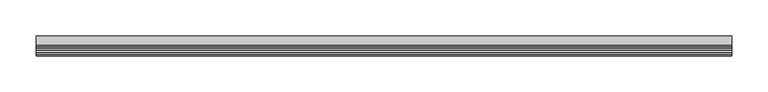
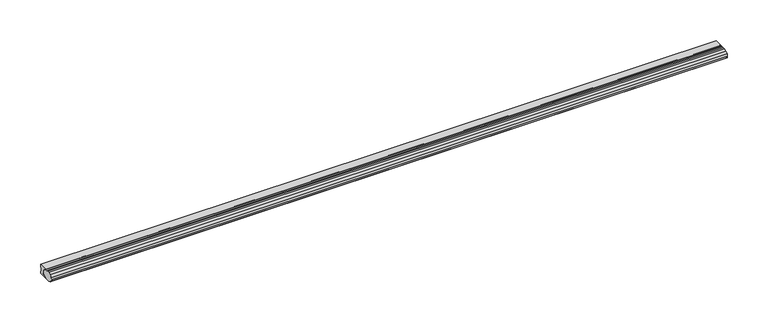
"""IFC4 building model written with IfcOpenShell, lengths in millimetres: proxy geometry, Generic Models 7:Generic Models 1:1:Generic Models 1:1 : Generic Models 7:Generic Models 1:337419:43 : Generic Models 7:Generic Models 1:1:Generic Models 1:1 : Generic Models 7:Generic Models 1:337419:306201."""

from ifc_helpers import new_model, si_unit, frame, origin, place, context, project, spatial, polyline, outline, extrude, source, transform, mapped, element, save


def generic_models_00966c09(model_context):
    return source(origin(), model_context, "Body", "SweptSolid", [
        extrude(outline(polyline([(-579016.3214511, 3715.5279199), (-579003.8663841, 3715.5279199), (-579004.6674366, 3713.4780806), (-579005.3332375, 3708.7889599), (-579004.6674366, 3704.0998393), (-579003.8663841, 3702.05), (-579016.3214511, 3702.05), (-579012.9398373, 3703.9237255), (-579010.8720803, 3706.5585721), (-579010.4416615, 3709.5423421), (-579011.7159161, 3712.4082526), (-579014.4954986, 3714.7079581), (-579016.3214511, 3715.5279199)])), frame((592776.2735285, 0.0, 0.0), z_axis=(1.0, 0.0, 0.0), x_axis=(0.0, 1.0, 0.0)), (0.0, 0.0, 1.0), 961.8131955),
        extrude(outline(polyline([(-579023.5876068, 3715.3589601), (-579021.3382673, 3715.5279199), (-579019.0889278, 3715.3589601), (-579015.0357581, 3714.057691), (-579012.2308776, 3711.7128851), (-579011.2298274, 3708.7889599), (-579012.2308776, 3705.8650348), (-579015.0357581, 3703.5202289), (-579019.0889278, 3702.2189598), (-579021.3382673, 3702.05), (-579023.5876068, 3702.2189598), (-579027.6407765, 3703.5202289), (-579030.4456569, 3705.8650348), (-579031.4467072, 3708.7889599), (-579030.4456569, 3711.7128851), (-579027.6407765, 3714.057691), (-579023.5876068, 3715.3589601)])), frame((592776.2735285, 0.0, 0.0), z_axis=(1.0, 0.0, 0.0), x_axis=(0.0, 1.0, 0.0)), (0.0, 0.0, 1.0), 961.8131955),
    ])


if __name__ == "__main__":
    model = new_model("IFC4")
    model_context = context("Model", 3, world=origin())
    ifc_project = project(units=[si_unit("LENGTHUNIT", "METRE", prefix="MILLI")], contexts=[model_context])
    site = spatial("IfcSite", under=ifc_project)
    building = spatial("IfcBuilding", under=site)
    placement = place(None, origin())
    generic_models_shape = generic_models_00966c09(model_context)
    element("IfcBuildingElementProxy", 1, Name="Generic Models 7:Generic Models 1:1:Generic Models 1:1 : Generic Models 7:Generic Models 1:337419:43 : Generic Models 7:Generic Models 1:1:Generic Models 1:1 : Generic Models 7:Generic Models 1:337419:306201", ObjectType="Generic Models 7:Generic Models 1:1:Generic Models 1:1 : Generic Models 7:Generic Models 1:337419:43 : Generic Models 7:Generic Models 1:1:Generic Models 1:1 : Generic Models 7:Generic Models 1:337419:306201", at=placement, inside=building, context=model_context, shape_type="MappedRepresentation", body=[
        mapped(generic_models_shape, transform((0.0, 0.0, 0.0), x_axis=(1.0, 0.0, 0.0), y_axis=(0.0, 1.0, 0.0), z_axis=(0.0, 0.0, 1.0))),
    ])
    save(model, "model.ifc")

# Revit data of these elements
# Type "Generic Models 7:Generic Models 1:1:Generic Models 1:1 : Generic Models 7:Generic Models 1:337419:43 : Generic Models 7:Generic Models 1:1:Generic Models 1:1 : Generic Models 7:Generic Models 1:337419:306201"
#   NameOverride = "Generic Models 7:Generic Models 1:1:Generic Models 1:1 : Generic Models 7:Generic Models 1:337419:306201"
#   ObjectTypeOverride = "Generic Models 1:1 : Generic Models 7:Generic Models 1:337419"
#   Reference = "Generic Models 1"
#   Tag = "306201"
# Element 1 (IfcBuildingElementProxy, "Generic Models 7:Generic Models 1:1:Generic Models 1:1 : Generic Models 7:Generic Models 1:337419:43 : Generic Models 7:Generic Models 1:1:Generic Models 1:1 : Generic Models 7:Generic Models 1:337419:306201")
#   Materials on its faces: "SEMI-RIGID EPOXY SEALANT W/ BACKROD (REMOVE TEMP. JOINT FORM)"
# Materials
#   "SEMI-RIGID EPOXY SEALANT W/ BACKROD (REMOVE TEMP. JOINT FORM)": class "Unassigned", colour RGB 120 120 120, transparency 0, Cost = 0
